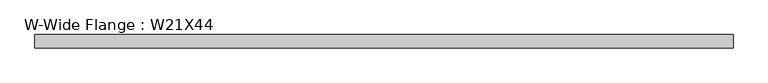
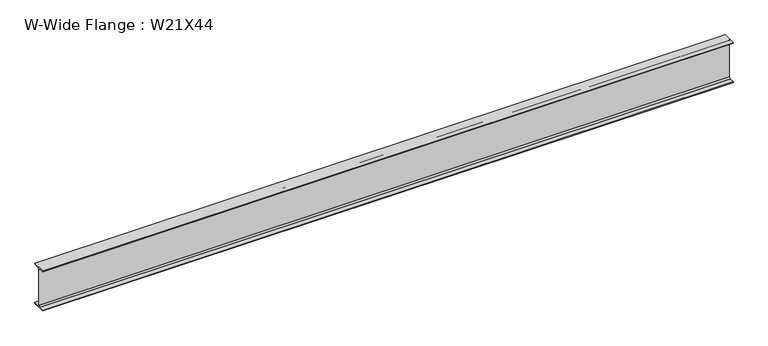
"""IFC4 building model written with IfcOpenShell, lengths in millimetres: beam geometry, W-Wide Flange : W21X44."""

from ifc_helpers import new_model, si_unit, point, frame, frame_2d, origin, place, context, project, spatial, polyline, circle_curve, trimmed, segment, composite_curve, outline, extrude, source, transform, mapped, element, save


def w_wide_flange_w21x44_87bcda2b(model_context):
    return source(origin(), model_context, "Body", "SweptSolid", [
        extrude(outline(composite_curve([segment(polyline([(82.55, -251.46), (82.55, -262.89), (-82.55, -262.89), (-82.55, -251.46), (-21.59, -251.46)]), True, "CONTINUOUS"), segment(trimmed(circle_curve(frame_2d((-21.59, -234.315)), 17.145), [point((-21.59, -251.46))], [point((-4.445, -234.315))], True, "CARTESIAN"), True, "CONTINUOUS"), segment(polyline([(-4.445, -234.315), (-4.445, 234.315)]), True, "CONTINUOUS"), segment(trimmed(circle_curve(frame_2d((-21.59, 234.315)), 17.145), [point((-4.445, 234.315))], [point((-21.59, 251.46))], True, "CARTESIAN"), True, "CONTINUOUS"), segment(polyline([(-21.59, 251.46), (-82.55, 251.46), (-82.55, 262.89), (82.55, 262.89), (82.55, 251.46), (21.59, 251.46)]), True, "CONTINUOUS"), segment(trimmed(circle_curve(frame_2d((21.59, 234.315)), 17.145), [point((21.59, 251.46))], [point((4.445, 234.315))], True, "CARTESIAN"), True, "CONTINUOUS"), segment(polyline([(4.445, 234.315), (4.445, -234.315)]), True, "CONTINUOUS"), segment(trimmed(circle_curve(frame_2d((21.59, -234.315)), 17.145), [point((4.445, -234.315))], [point((21.59, -251.46))], True, "CARTESIAN"), True, "CONTINUOUS"), segment(polyline([(21.59, -251.46), (82.55, -251.46)]), True, "CONTINUOUS")], self_intersect=False)), frame((-4220.21, 0.0, 0.0), z_axis=(1.0, 0.0, 0.0), x_axis=(0.0, 1.0, 0.0)), (0.0, 0.0, 1.0), 8544.56),
    ])


if __name__ == "__main__":
    model = new_model("IFC4")
    model_context = context("Model", 3, world=origin())
    ifc_project = project(units=[si_unit("LENGTHUNIT", "METRE", prefix="MILLI")], contexts=[model_context])
    site = spatial("IfcSite", under=ifc_project)
    building = spatial("IfcBuilding", under=site)
    placement = place(None, origin())
    w_wide_flange_w21x44_shape = w_wide_flange_w21x44_87bcda2b(model_context)
    element("IfcBeam", 1, ObjectType="W-Wide Flange : W21X44", at=placement, inside=building, context=model_context, shape_type="MappedRepresentation", body=[
        mapped(w_wide_flange_w21x44_shape, transform((0.0, 0.0, 0.0), x_axis=(1.0, 0.0, 0.0), y_axis=(0.0, 1.0, 0.0), z_axis=(0.0, 0.0, 1.0))),
    ])
    save(model, "model.ifc")

# Revit data of these elements
# Type "W-Wide Flange : W21X44"
#   Assembly Code = "B10"
#   W = 44
#   Start Extension Calculation [instance default] = 10' - 0"
#   Start Extension [instance default] = -0' - 0 1/2"
#   End Extension Calculation [instance default] = 10' - 0"
#   End Extension [instance default] = -0' - 0 1/2"
#   Length [instance default] = 5' - 0"
#   bf = 0' - 6 1/2"
#   d = 1' - 8.7"
#   k = 0' - 1 1/8"
#   k2 = 0' - 0.675"
#   tf = 0' - 0.45"
#   tw = 0' - 0.35"
#   A = 0.0902778 SF
#   Beam Material [instance default] = Metal - Steel - ASTM A992
# Element 1 (IfcBeam, "W-Wide Flange : W21X44")
#   Materials on its faces: "Metal - Steel - ASTM A992"
# Materials
#   "Metal - Steel - ASTM A992": class "Metal", colour RGB 128 0 0, transparency 0
